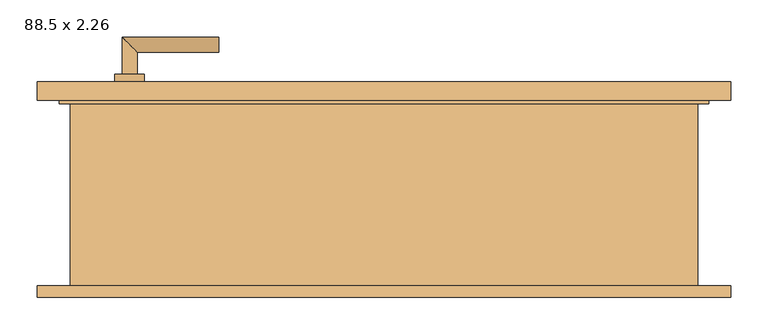
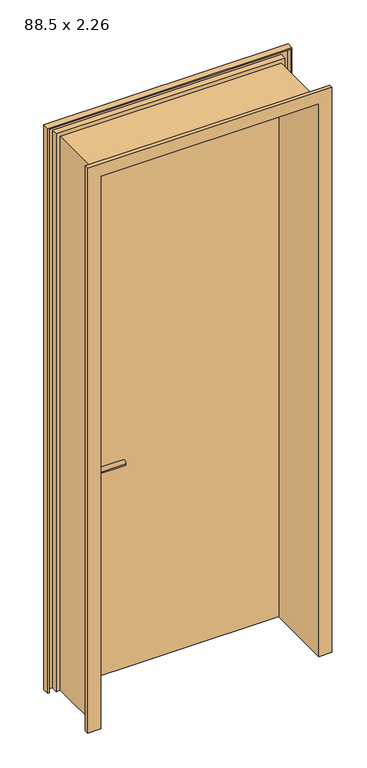
"""IFC4 building model written with IfcOpenShell, lengths in millimetres: door geometry, Drehflügel 1-flg - Stahlzarge : 88.5 x 2.26."""

import ifcopenshell
import ifcopenshell.guid

model = None  # the IFC model being written
_history = None  # IfcOwnerHistory: only IFC2X3 demands one
_inside = {}  # id of a spatial element -> (the spatial element, [elements in it])
_under = {}  # id of a project, library or spatial element -> (it, [spatial elements below it])
_declared = {}  # id of a project -> (the project, [libraries it declares])
_typed = {}  # id of a type object -> (the type object, [elements of that type])
_made_of = {}  # id of a material, layer set ... -> (it, [elements and type objects made of it])


def new_model(schema):
    """Start an empty IFC model of exactly this schema.

    Asked for "IFC4X3", IfcOpenShell would pick the latest addendum, in which some entities
    have other attributes; the version numbers below select the first issue.
    IFC2X3 requires an IfcOwnerHistory on every rooted entity: one is made here for all.
    """
    global model, _history
    if schema == "IFC4X3":
        model = ifcopenshell.file(schema_version=(4, 3, 0, 0))
    else:
        model = ifcopenshell.file(schema=schema)
    _inside.clear()
    _under.clear()
    _declared.clear()
    _typed.clear()
    _made_of.clear()
    _history = None
    if model.schema == "IFC2X3":
        org = make("IfcOrganization", Name="unknown")
        user = make(
            "IfcPersonAndOrganization",
            ThePerson=make("IfcPerson", FamilyName="unknown"),
            TheOrganization=org,
        )
        app = make(
            "IfcApplication",
            ApplicationDeveloper=org,
            Version="unknown",
            ApplicationFullName="unknown",
            ApplicationIdentifier="unknown",
        )
        _history = make(
            "IfcOwnerHistory",
            OwningUser=user,
            OwningApplication=app,
            ChangeAction="ADDED",
            CreationDate=0,
        )
    return model


def make(cls, **values):
    """One entity of the class cls with the attributes given. An attribute that is None is left unset."""
    return model.create_entity(
        cls, **{name: value for name, value in values.items() if value is not None}
    )


def rooted(cls, **values):
    """An entity with a GlobalId (a new one), such as an element, a storey or a relation."""
    return make(cls, GlobalId=ifcopenshell.guid.new(), OwnerHistory=_history, **values)


def si_unit(unit_type, name, prefix=None):
    """IfcSIUnit, for example si_unit("LENGTHUNIT", "METRE", prefix="MILLI")."""
    return make("IfcSIUnit", UnitType=unit_type, Prefix=prefix, Name=name)


def assignment(units):
    """IfcUnitAssignment: the units of a project."""
    return None if units is None else make("IfcUnitAssignment", Units=units)


def point(xyz):
    """IfcCartesianPoint."""
    return None if xyz is None else make("IfcCartesianPoint", Coordinates=xyz)


def direction(xyz):
    """IfcDirection."""
    return None if xyz is None else make("IfcDirection", DirectionRatios=xyz)


def frame(location, z_axis=None, x_axis=None):
    """IfcAxis2Placement3D, a coordinate frame: its origin and axes. An axis left out is left unset."""
    return make(
        "IfcAxis2Placement3D",
        Location=point(location),
        Axis=direction(z_axis),
        RefDirection=direction(x_axis),
    )


def frame_2d(location, x_axis=None):
    """IfcAxis2Placement2D, a coordinate frame in the plane: its origin and x axis."""
    return make(
        "IfcAxis2Placement2D", Location=point(location), RefDirection=direction(x_axis)
    )


def origin():
    """The frame at (0, 0, 0) with its axes left unset."""
    return frame((0.0, 0.0, 0.0))


def origin_with_axes():
    """The frame at (0, 0, 0) with the z axis (0, 0, 1) and the x axis (1, 0, 0) written out."""
    return frame((0.0, 0.0, 0.0), z_axis=(0.0, 0.0, 1.0), x_axis=(1.0, 0.0, 0.0))


def place(relative_to, where):
    """IfcLocalPlacement: puts the frame where relative to a parent placement (None: the world)."""
    return make(
        "IfcLocalPlacement", PlacementRelTo=relative_to, RelativePlacement=where
    )


def context(
    kind, dimensions, precision=None, world=None, true_north=None, identifier=None
):
    """IfcGeometricRepresentationContext, for example the 3D "Model" context."""
    return make(
        "IfcGeometricRepresentationContext",
        ContextIdentifier=identifier,
        ContextType=kind,
        CoordinateSpaceDimension=dimensions,
        Precision=precision,
        WorldCoordinateSystem=world,
        TrueNorth=true_north,
    )


def project(units=None, contexts=None):
    """IfcProject with its units and contexts."""
    return rooted(
        "IfcProject",
        Name="project",
        RepresentationContexts=contexts,
        UnitsInContext=assignment(units),
    )


def spatial(cls, under=None, at=None, **own):
    """A site, building, storey or space (cls), placed at a placement, below another one or the project."""
    s = rooted(cls, ObjectPlacement=at, **own)
    if under is not None:
        _under.setdefault(under.id(), (under, []))[1].append(s)
    return s


def polyline(points):
    """IfcPolyline through the points."""
    return make("IfcPolyline", Points=[point(p) for p in points])


def circle_curve(where, radius):
    """IfcCircle in the frame where."""
    return make("IfcCircle", Position=where, Radius=radius)


def ellipse_curve(where, semi_axis1, semi_axis2):
    """IfcEllipse in the frame where."""
    return make(
        "IfcEllipse", Position=where, SemiAxis1=semi_axis1, SemiAxis2=semi_axis2
    )


def trimmed(basis, trim1, trim2, sense, master):
    """IfcTrimmedCurve: the piece of a basis curve between two trims."""
    return make(
        "IfcTrimmedCurve",
        BasisCurve=basis,
        Trim1=trim1,
        Trim2=trim2,
        SenseAgreement=sense,
        MasterRepresentation=master,
    )


def segment(curve, same_sense, transition):
    """IfcCompositeCurveSegment."""
    return make(
        "IfcCompositeCurveSegment",
        Transition=transition,
        SameSense=same_sense,
        ParentCurve=curve,
    )


def composite_curve(segments, self_intersect=None):
    """IfcCompositeCurve: segments joined end to end."""
    return make("IfcCompositeCurve", Segments=segments, SelfIntersect=self_intersect)


def outline(outer, holes=None, kind="AREA"):
    """IfcArbitraryClosedProfileDef: a profile drawn as a closed curve; with holes, ...WithVoids."""
    if holes is None:
        return make("IfcArbitraryClosedProfileDef", ProfileType=kind, OuterCurve=outer)
    return make(
        "IfcArbitraryProfileDefWithVoids",
        ProfileType=kind,
        OuterCurve=outer,
        InnerCurves=holes,
    )


def extrude(swept, where, along, depth):
    """IfcExtrudedAreaSolid: the profile swept, set in the frame where, extruded along a direction by depth."""
    return make(
        "IfcExtrudedAreaSolid",
        SweptArea=swept,
        Position=where,
        ExtrudedDirection=direction(along),
        Depth=depth,
    )


def faces_of(points, faces, orient=None, outer=None):
    """IfcFace entities. A face is a list of loops; a loop is a list of indices into points, from 0.

    orient and outer hold one flag for each loop. By default every Orientation is true, the
    first loop of a face is its IfcFaceOuterBound and the others are IfcFaceBound.
    """
    made = []
    for i, loops in enumerate(faces):
        bounds = []
        for j, loop in enumerate(loops):
            is_outer = j == 0 if outer is None else outer[i][j]
            bounds.append(
                make(
                    "IfcFaceOuterBound" if is_outer else "IfcFaceBound",
                    Bound=make("IfcPolyLoop", Polygon=[points[k] for k in loop]),
                    Orientation=True if orient is None else orient[i][j],
                )
            )
        made.append(make("IfcFace", Bounds=bounds))
    return made


def faceted_brep(points, faces, orient=None, outer=None, voids=None):
    """IfcFacetedBrep: a solid bounded by flat faces; with voids (closed shells), ...WithVoids."""
    shared = [point(p) for p in points]
    hull = make("IfcClosedShell", CfsFaces=faces_of(shared, faces, orient, outer))
    if voids is None:
        return make("IfcFacetedBrep", Outer=hull)
    return make(
        "IfcFacetedBrepWithVoids",
        Outer=hull,
        Voids=[
            make(cls, CfsFaces=faces_of(shared, fs, o, b)) for cls, fs, o, b in voids
        ],
    )


def shape(context_of_items, identifier, shape_type, items):
    """IfcShapeRepresentation: the items that make up one representation, for example the "Body"."""
    return make(
        "IfcShapeRepresentation",
        ContextOfItems=context_of_items,
        RepresentationIdentifier=identifier,
        RepresentationType=shape_type,
        Items=items,
    )


def source(mapping_origin, context_of_items, identifier, shape_type, items):
    """IfcRepresentationMap: a shape defined once, which mapped items show again and again."""
    return make(
        "IfcRepresentationMap",
        MappingOrigin=mapping_origin,
        MappedRepresentation=shape(context_of_items, identifier, shape_type, items),
    )


def transform(
    local_origin,
    x_axis=None,
    y_axis=None,
    z_axis=None,
    scale=None,
    scale2=None,
    scale3=None,
    uniform=True,
):
    """IfcCartesianTransformationOperator3D, or its non-uniform kind. x_axis, y_axis, z_axis: its Axis1, 2, 3."""
    if uniform:
        return make(
            "IfcCartesianTransformationOperator3D",
            Axis1=direction(x_axis),
            Axis2=direction(y_axis),
            LocalOrigin=point(local_origin),
            Scale=scale,
            Axis3=direction(z_axis),
        )
    return make(
        "IfcCartesianTransformationOperator3DnonUniform",
        Axis1=direction(x_axis),
        Axis2=direction(y_axis),
        LocalOrigin=point(local_origin),
        Scale=scale,
        Axis3=direction(z_axis),
        Scale2=scale2,
        Scale3=scale3,
    )


def mapped(mapping_source, mapping_target):
    """IfcMappedItem: shows the shape of a source again, moved by a transform."""
    return make(
        "IfcMappedItem", MappingSource=mapping_source, MappingTarget=mapping_target
    )


def made_of(thing, what):
    """Note that an element or type object is made of a material, layer set ...; save() writes the relation."""
    if what is not None:
        _made_of.setdefault(what.id(), (what, []))[1].append(thing)
    return thing


def element(
    cls,
    number,
    at=None,
    inside=None,
    cuts=None,
    type_object=None,
    material=None,
    context=None,
    identifier="Body",
    shape_type=None,
    held_by="IfcProductDefinitionShape",
    body=None,
    shapes=None,
    **own,
):
    """One element of the class cls, such as IfcWall. Its Tag is "e" and its number.

    at: its placement. inside: the storey or other place that contains it. cuts: it is an
    opening in that element (IfcRelVoidsElement). A single representation is given by context,
    identifier, shape_type and body (its items); several are given by shapes. held_by: the class
    of the entity that holds the representations. save() writes the other relations.
    """
    e = rooted(cls, Tag="e%d" % number, ObjectPlacement=at, **own)
    if body is not None:
        shapes = [shape(context, identifier, shape_type, body)]
    if shapes is not None:
        e.Representation = make(held_by, Representations=shapes)
    if inside is not None:
        _inside.setdefault(inside.id(), (inside, []))[1].append(e)
    if cuts is not None:
        rooted(
            "IfcRelVoidsElement", RelatingBuildingElement=cuts, RelatedOpeningElement=e
        )
    if type_object is not None:
        _typed.setdefault(type_object.id(), (type_object, []))[1].append(e)
    return made_of(e, material)


def aggregate(whole, parts):
    """IfcRelAggregates: a whole, such as a stair, and the parts it consists of."""
    return rooted("IfcRelAggregates", RelatingObject=whole, RelatedObjects=parts)


def save(model, path):
    """Write the relations noted so far, then the file.

    IfcRelAggregates (storeys below a building ...), IfcRelContainedInSpatialStructure (elements
    in a storey), IfcRelDefinesByType, IfcRelAssociatesMaterial and IfcRelDeclares: one each for
    every whole, place, type object, material and project.
    """
    for whole, parts in _under.values():
        aggregate(whole, parts)
    for where, things in _inside.values():
        rooted(
            "IfcRelContainedInSpatialStructure",
            RelatedElements=things,
            RelatingStructure=where,
        )
    for kind, things in _typed.values():
        rooted("IfcRelDefinesByType", RelatedObjects=things, RelatingType=kind)
    for what, things in _made_of.values():
        rooted("IfcRelAssociatesMaterial", RelatedObjects=things, RelatingMaterial=what)
    for by, libraries in _declared.values():
        rooted("IfcRelDeclares", RelatingContext=by, RelatedDefinitions=libraries)
    model.write(path)


def plane_surface(at):
    """IfcPlane: the flat surface through the origin of the frame at, square to its z axis."""
    return make("IfcPlane", Position=at)


def cylinder_surface(at, radius):
    """IfcCylindricalSurface: all points at the distance radius from the z axis of the frame at."""
    return make("IfcCylindricalSurface", Position=at, Radius=radius)


def advanced_brep(points, edges, surfaces, faces):
    """IfcAdvancedBrep: a solid bounded by faces that lie on surfaces and meet in shared edges.

    An edge is (start, end): straight between two places in points (the first is 0);
    or (start, end, curve); or (start, end, curve, False) where it runs against its curve.
    A face is (place in surfaces, loops), or (place, loops, False) where it looks against
    its surface's normal. A loop lists edges by number (the first is 1), with a minus sign
    where the edge is run from its end to its start. The first loop is the outer one.
    """
    corners = [point(p) for p in points]
    vertices = [make("IfcVertexPoint", VertexGeometry=c) for c in corners]
    made = []
    for start, end, *more in edges:
        made.append(
            make(
                "IfcEdgeCurve",
                EdgeStart=vertices[start],
                EdgeEnd=vertices[end],
                EdgeGeometry=more[0] if more else make("IfcPolyline", Points=[corners[start], corners[end]]),
                SameSense=more[1] if len(more) > 1 else True,
            )
        )
    hull = []
    for where, loops, *sense in faces:
        bounds = []
        for j, loop in enumerate(loops):
            ring = [make("IfcOrientedEdge", EdgeElement=made[abs(k) - 1], Orientation=k > 0) for k in loop]
            bounds.append(
                make(
                    "IfcFaceOuterBound" if j == 0 else "IfcFaceBound",
                    Bound=make("IfcEdgeLoop", EdgeList=ring),
                    Orientation=True,
                )
            )
        hull.append(make("IfcAdvancedFace", Bounds=bounds, FaceSurface=surfaces[where], SameSense=sense[0] if sense else True))
    return make("IfcAdvancedBrep", Outer=make("IfcClosedShell", CfsFaces=hull))


def door_88_5_x_2_26_0a08d8ab(model_context):
    return source(origin(), model_context, "Body", "SolidModel", [
        advanced_brep(
        [(-352.5, 114.4346141, 900.0), (-332.5, 114.4346141, 900.0), (-352.5, 44.4346141, 900.0), (-332.5, 64.4346141, 900.0), (-222.5, 44.4346141, 900.0), (-222.5, 64.4346141, 900.0)],
        [
            (0, 1, circle_curve(frame((-342.5, 114.4346141, 900.0), z_axis=(0.0, 1.0, 0.0), x_axis=(1.0, 0.0, 0.0)), 10.0)),
            (1, 0, circle_curve(frame((-342.5, 114.4346141, 900.0), z_axis=(0.0, 1.0, 0.0), x_axis=(1.0, 0.0, 0.0)), 10.0)),
            (0, 2),
            (2, 3, ellipse_curve(frame((-342.5, 54.4346141, 900.0), z_axis=(-0.7071067811865385, 0.7071067811865565, 0.0), x_axis=(0.7071067811865563, 0.7071067811865386, 0.0)), 14.1421356, 10.0)),
            (3, 1),
            (3, 2, ellipse_curve(frame((-342.5, 54.4346141, 900.0), z_axis=(-0.7071067811865385, 0.7071067811865565, 0.0), x_axis=(0.7071067811865563, 0.7071067811865386, 0.0)), 14.1421356, 10.0)),
            (4, 5, circle_curve(frame((-222.5, 54.4346141, 900.0), z_axis=(1.0, 0.0, 0.0), x_axis=(0.0, 1.0, 0.0)), 10.0)),
            (5, 4, circle_curve(frame((-222.5, 54.4346141, 900.0), z_axis=(1.0, 0.0, 0.0), x_axis=(0.0, 1.0, 0.0)), 10.0)),
            (2, 4),
            (5, 3),
        ],
        [
            plane_surface(frame((-342.5, 114.4346141, -387.7526403), z_axis=(0.0, 1.0, 0.0), x_axis=(0.0, 0.0, 1.0))),
            cylinder_surface(frame((-342.5, 114.4346141, 900.0), z_axis=(0.0, 1.0, 0.0), x_axis=(1.0, 0.0, 0.0)), 10.0),
            plane_surface(frame((-222.5, 54.4346141, -387.7526403), z_axis=(1.0, 0.0, 0.0), x_axis=(0.0, 0.0, 1.0))),
            cylinder_surface(frame((-342.5, 54.4346141, 900.0), z_axis=(-1.0, 0.0, 0.0), x_axis=(0.0, 1.0, 0.0)), 10.0),
        ],
        [
            (0, [[1, 2]]),
            (1, [[-1, 3, 4, 5]]),
            (1, [[-2, -5, 6, -3]]),
            (2, [[7, 8]]),
            (3, [[-4, 9, -8, 10]]),
            (3, [[-6, -10, -7, -9]]),
        ],
    ),
        advanced_brep(
        [(-332.5, 174.4346141, 900.0), (-352.5, 174.4346141, 900.0), (-332.5, 204.4346141, 900.0), (-352.5, 224.4346141, 900.0), (-222.5, 204.4346141, 900.0), (-222.5, 224.4346141, 900.0)],
        [
            (0, 1, circle_curve(frame((-342.5, 174.4346141, 900.0), z_axis=(0.0, -1.0, 0.0), x_axis=(-1.0, 0.0, 0.0)), 10.0)),
            (1, 0, circle_curve(frame((-342.5, 174.4346141, 900.0), z_axis=(0.0, -1.0, 0.0), x_axis=(-1.0, 0.0, 0.0)), 10.0)),
            (0, 2),
            (2, 3, ellipse_curve(frame((-342.5, 214.4346141, 900.0), z_axis=(-0.7071067811865475, -0.7071067811865475, 0.0), x_axis=(0.7071067811865474, -0.7071067811865476, 0.0)), 14.1421356, 10.0)),
            (3, 1),
            (3, 2, ellipse_curve(frame((-342.5, 214.4346141, 900.0), z_axis=(-0.7071067811865475, -0.7071067811865475, 0.0), x_axis=(0.7071067811865474, -0.7071067811865476, 0.0)), 14.1421356, 10.0)),
            (4, 5, circle_curve(frame((-222.5, 214.4346141, 900.0), z_axis=(1.0, 0.0, 0.0), x_axis=(0.0, 1.0, 0.0)), 10.0)),
            (5, 4, circle_curve(frame((-222.5, 214.4346141, 900.0), z_axis=(1.0, 0.0, 0.0), x_axis=(0.0, 1.0, 0.0)), 10.0)),
            (2, 4),
            (5, 3),
        ],
        [
            plane_surface(frame((-342.5, 174.4346141, -387.7526403), z_axis=(0.0, -1.0, 0.0), x_axis=(0.0, 0.0, 1.0))),
            cylinder_surface(frame((-342.5, 174.4346141, 900.0), z_axis=(0.0, -1.0, 0.0), x_axis=(-1.0, 0.0, 0.0)), 10.0),
            plane_surface(frame((-222.5, 214.4346141, -387.7526403), z_axis=(1.0, 0.0, 0.0), x_axis=(0.0, 0.0, 1.0))),
            cylinder_surface(frame((-342.5, 214.4346141, 900.0), z_axis=(-1.0, 0.0, 0.0), x_axis=(0.0, 1.0, 0.0)), 10.0),
        ],
        [
            (0, [[1, 2]]),
            (1, [[-1, 3, 4, 5]]),
            (1, [[-2, -5, 6, -3]]),
            (2, [[7, 8]]),
            (3, [[-4, 9, -8, 10]]),
            (3, [[-6, -10, -7, -9]]),
        ],
    ),
        extrude(outline(composite_curve([segment(trimmed(circle_curve(frame_2d((900.0, -342.5)), 20.0), [point((900.0, -362.5))], [point((900.0, -322.5))], False, "CARTESIAN"), True, "CONTINUOUS"), segment(trimmed(circle_curve(frame_2d((900.0, -342.5)), 20.0), [point((900.0, -322.5))], [point((900.0, -362.5))], False, "CARTESIAN"), True, "CONTINUOUS")], self_intersect=False)), frame((0.0, 104.4346141, 0.0), z_axis=(0.0, 1.0, 0.0), x_axis=(0.0, 0.0, 1.0)), (0.0, 0.0, 1.0), 10.0),
        extrude(outline(composite_curve([segment(trimmed(circle_curve(frame_2d((900.0, -342.5)), 20.0), [point((900.0, -362.5))], [point((900.0, -322.5))], False, "CARTESIAN"), True, "CONTINUOUS"), segment(trimmed(circle_curve(frame_2d((900.0, -342.5)), 20.0), [point((900.0, -322.5))], [point((900.0, -362.5))], False, "CARTESIAN"), True, "CONTINUOUS")], self_intersect=False)), frame((0.0, 164.4346141, 0.0), z_axis=(0.0, 1.0, 0.0), x_axis=(0.0, 0.0, 1.0)), (0.0, 0.0, 1.0), 10.0),
        extrude(outline(polyline([(432.5, 139.4346141), (-432.5, 139.4346141), (-432.5, 164.4346141), (432.5, 164.4346141), (432.5, 139.4346141)])), origin_with_axes(), (0.0, 0.0, 1.0), 2250.0),
        faceted_brep([(466.9603207, -125.5653859, 0.0), (417.5, -125.5653859, 0.0), (417.5, 139.4346141, 0.0), (432.5, 139.4346141, 0.0), (432.5, 164.4346141, 0.0), (466.9603207, 164.4346141, 0.0), (466.9603207, 139.4346141, 0.0), (461.9603207, 139.4346141, 0.0), (461.9603207, 159.4346141, 0.0), (437.5, 159.4346141, 0.0), (437.5, 134.4346141, 0.0), (422.5, 134.4346141, 0.0), (422.5, -120.5653859, 0.0), (461.9603207, -120.5653859, 0.0), (461.9603207, -110.5653859, 0.0), (466.9603207, -110.5653859, 0.0), (466.9603207, -125.5653859, 2284.4603207), (-466.9603207, -125.5653859, 2284.4603207), (-466.9603207, -125.5653859, 0.0), (-417.5, -125.5653859, 0.0), (-417.5, -125.5653859, 2235.0), (417.5, -125.5653859, 2235.0), (417.5, 139.4346141, 2235.0), (-417.5, 139.4346141, 2235.0), (-417.5, 139.4346141, 0.0), (-432.5, 139.4346141, 0.0), (-432.5, 139.4346141, 2250.0), (432.5, 139.4346141, 2250.0), (432.5, 164.4346141, 2250.0), (-432.5, 164.4346141, 2250.0), (-432.5, 164.4346141, 0.0), (-466.9603207, 164.4346141, 0.0), (-466.9603207, 164.4346141, 2284.4603207), (466.9603207, 164.4346141, 2284.4603207), (466.9603207, 139.4346141, 2284.4603207), (-466.9603207, 139.4346141, 2284.4603207), (-466.9603207, 139.4346141, 0.0), (-461.9603207, 139.4346141, 0.0), (-461.9603207, 139.4346141, 2279.4603207), (461.9603207, 139.4346141, 2279.4603207), (461.9603207, 159.4346141, 2279.4603207), (-461.9603207, 159.4346141, 2279.4603207), (-461.9603207, 159.4346141, 0.0), (-437.5, 159.4346141, 0.0), (-437.5, 159.4346141, 2255.0), (437.5, 159.4346141, 2255.0), (437.5, 134.4346141, 2255.0), (-437.5, 134.4346141, 2255.0), (-437.5, 134.4346141, 0.0), (-422.5, 134.4346141, 0.0), (-422.5, 134.4346141, 2240.0), (422.5, 134.4346141, 2240.0), (422.5, -120.5653859, 2240.0), (-422.5, -120.5653859, 2240.0), (-422.5, -120.5653859, 0.0), (-461.9603207, -120.5653859, 0.0), (-461.9603207, -120.5653859, 2279.4603207), (461.9603207, -120.5653859, 2279.4603207), (461.9603207, -110.5653859, 2279.4603207), (-461.9603207, -110.5653859, 2279.4603207), (-461.9603207, -110.5653859, 0.0), (-466.9603207, -110.5653859, 0.0), (-466.9603207, -110.5653859, 2284.4603207), (466.9603207, -110.5653859, 2284.4603207)], [[[0, 1, 2, 3, 4, 5, 6, 7, 8, 9, 10, 11, 12, 13, 14, 15]], [[1, 0, 16, 17, 18, 19, 20, 21]], [[2, 1, 21, 22]], [[3, 2, 22, 23, 24, 25, 26, 27]], [[4, 3, 27, 28]], [[5, 4, 28, 29, 30, 31, 32, 33]], [[6, 5, 33, 34]], [[7, 6, 34, 35, 36, 37, 38, 39]], [[8, 7, 39, 40]], [[9, 8, 40, 41, 42, 43, 44, 45]], [[10, 9, 45, 46]], [[11, 10, 46, 47, 48, 49, 50, 51]], [[12, 11, 51, 52]], [[13, 12, 52, 53, 54, 55, 56, 57]], [[14, 13, 57, 58]], [[15, 14, 58, 59, 60, 61, 62, 63]], [[0, 15, 63, 16]], [[17, 62, 61, 18]], [[18, 61, 60, 55, 54, 49, 48, 43, 42, 37, 36, 31, 30, 25, 24, 19]], [[23, 20, 19, 24]], [[29, 26, 25, 30]], [[35, 32, 31, 36]], [[41, 38, 37, 42]], [[47, 44, 43, 48]], [[53, 50, 49, 54]], [[59, 56, 55, 60]], [[22, 21, 20, 23]], [[28, 27, 26, 29]], [[34, 33, 32, 35]], [[40, 39, 38, 41]], [[46, 45, 44, 47]], [[52, 51, 50, 53]], [[58, 57, 56, 59]], [[16, 63, 62, 17]]]),
    ])


if __name__ == "__main__":
    model = new_model("IFC4")
    model_context = context("Model", 3, world=origin())
    ifc_project = project(units=[si_unit("LENGTHUNIT", "METRE", prefix="MILLI")], contexts=[model_context])
    site = spatial("IfcSite", under=ifc_project)
    building = spatial("IfcBuilding", under=site)
    placement = place(None, origin())
    door_88_5_x_2_26_shape = door_88_5_x_2_26_0a08d8ab(model_context)
    element("IfcDoor", 1, ObjectType="Drehflügel 1-flg - Stahlzarge : 88.5 x 2.26", at=placement, inside=building, context=model_context, shape_type="MappedRepresentation", body=[
        mapped(door_88_5_x_2_26_shape, transform((0.0, 0.0, 0.0), x_axis=(1.0, 0.0, 0.0), y_axis=(0.0, 1.0, 0.0), z_axis=(0.0, 0.0, 1.0))),
    ])
    save(model, "model.ifc")

# Revit data of these elements
# Type "Drehflügel 1-flg - Stahlzarge : 88.5 x 2.26"
#   Construction Type Id = "MDOOR"
#   Type Mark = "20"
#   Operation = "SingleSwingRight"
#   Keynote = "16.03"
#   Analytic Construction = "Metall"
#   Thermal Resistance (R) = 0.270117 (m²·K)/W
#   Heat Transfer Coefficient (U) = 3.7021 W/(m²·K)
#   Rough Width = 0.885 m
#   Rough Height [instance default] = 2.360 m
#   Höhe Türgriff [instance default] = 0.900 m
#   Height = 2.260 m
#   Fußbodenaufbau [instance default] = 0.100 m
#   Width = 0.885 m
#   Sichtbarkeit Sturzlinien [instance default] = yes
#   Türgriff auswählen [instance default] = element 221079
#   Türgriff [instance default] = none
#   Türflügel [instance default] = none
#   Rahmen/Pfosten [instance default] = Metall - Lackiert - Grau
#   Visual Light Transmittance = 0
#   Solar Heat Gain Coefficient = 0
#   Function = (empty or 0)
#   Wall Closure = (empty or 0)
# Element 1 (IfcDoor, "Drehflügel 1-flg - Stahlzarge : 88.5 x 2.26")
#   Rough Height = 2.260 m
#   Fußbodenaufbau = 0.000 m
#   Materials on its faces: "Metall - Lackiert - Grau", "Metall - Chrom", "Holz - Birke"
# Materials
#   "Metall - Lackiert - Grau": class "Farbe 1", colour RGB 98 98 98, transparency 0, Cost = 0
#   "Metall - Chrom": class "Metall", colour RGB 247 247 247, transparency 0, Cost = 0
#   "Holz - Birke": class "Holz", colour RGB 213 164 103, transparency 0, Cost = 0
